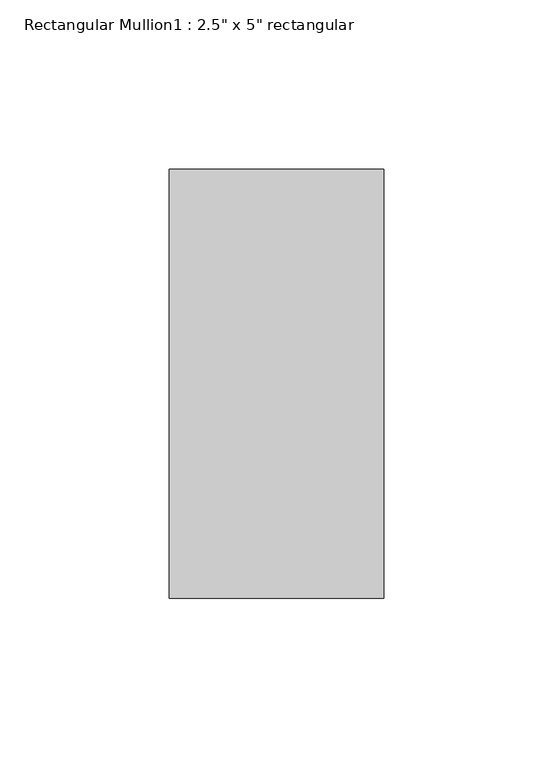
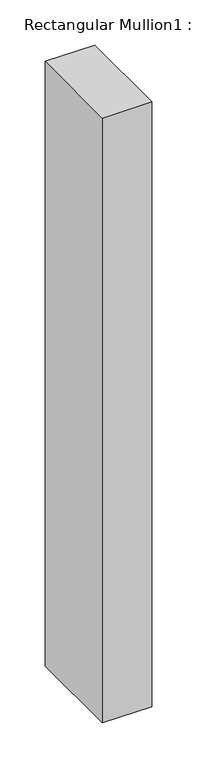
"""IFC4 building model written with IfcOpenShell, lengths in millimetres: member geometry."""

from ifc_helpers import new_model, si_unit, frame, origin, place, context, project, spatial, polyline, outline, extrude, source, transform, mapped, element, save


def member_c17f1be2(model_context):
    return source(origin(), model_context, "Body", "SweptSolid", [
        extrude(outline(polyline([(0.0, 63.5), (0.0, -63.5), (-63.5, -63.5), (-63.5, 63.5), (0.0, 63.5)])), frame((0.0, 0.0, -819.15), z_axis=(0.0, 0.0, 1.0), x_axis=(1.0, 0.0, 0.0)), (0.0, 0.0, 1.0), 819.15),
    ])


if __name__ == "__main__":
    model = new_model("IFC4")
    model_context = context("Model", 3, world=origin())
    ifc_project = project(units=[si_unit("LENGTHUNIT", "METRE", prefix="MILLI")], contexts=[model_context])
    site = spatial("IfcSite", under=ifc_project)
    building = spatial("IfcBuilding", under=site)
    placement = place(None, origin())
    member_shape = member_c17f1be2(model_context)
    element("IfcMember", 1, ObjectType="Rectangular Mullion1 : 2.5\" x 5\" rectangular", at=placement, inside=building, context=model_context, shape_type="MappedRepresentation", body=[
        mapped(member_shape, transform((0.0, 0.0, 0.0), x_axis=(1.0, 0.0, 0.0), y_axis=(0.0, 1.0, 0.0), z_axis=(0.0, 0.0, 1.0))),
    ])
    save(model, "model.ifc")

# Revit data of these elements
# Type "Rectangular Mullion1 : 2.5\" x 5\" rectangular"
#   built-in parameter 1007304 = 0.416667 (stored number, unit not read)
#   built-in parameter 1007301 = 0.104167 (stored number, unit not read)
#   built-in parameter 1007300 = 0.104167 (stored number, unit not read)
# Element 1 (IfcMember, "Rectangular Mullion1 : 2.5\" x 5\" rectangular")
#   Materials on its faces: "support-frame"
# Materials
#   "support-frame": class "Unassigned", colour RGB 233 233 233, transparency 0, Cost = 0
